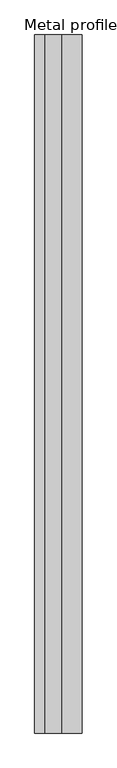
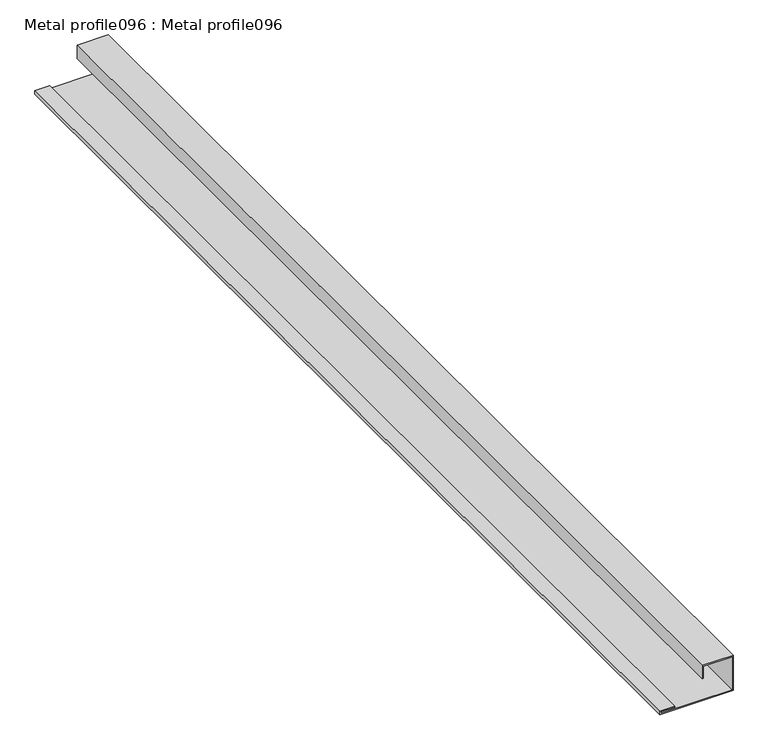
"""IFC4 building model written with IfcOpenShell, lengths in millimetres: proxy geometry, Metal profile096 : Metal profile096."""

import ifcopenshell
import ifcopenshell.guid

model = None  # the IFC model being written
_history = None  # IfcOwnerHistory: only IFC2X3 demands one
_inside = {}  # id of a spatial element -> (the spatial element, [elements in it])
_under = {}  # id of a project, library or spatial element -> (it, [spatial elements below it])
_declared = {}  # id of a project -> (the project, [libraries it declares])
_typed = {}  # id of a type object -> (the type object, [elements of that type])
_made_of = {}  # id of a material, layer set ... -> (it, [elements and type objects made of it])


def new_model(schema):
    """Start an empty IFC model of exactly this schema.

    Asked for "IFC4X3", IfcOpenShell would pick the latest addendum, in which some entities
    have other attributes; the version numbers below select the first issue.
    IFC2X3 requires an IfcOwnerHistory on every rooted entity: one is made here for all.
    """
    global model, _history
    if schema == "IFC4X3":
        model = ifcopenshell.file(schema_version=(4, 3, 0, 0))
    else:
        model = ifcopenshell.file(schema=schema)
    _inside.clear()
    _under.clear()
    _declared.clear()
    _typed.clear()
    _made_of.clear()
    _history = None
    if model.schema == "IFC2X3":
        org = make("IfcOrganization", Name="unknown")
        user = make(
            "IfcPersonAndOrganization",
            ThePerson=make("IfcPerson", FamilyName="unknown"),
            TheOrganization=org,
        )
        app = make(
            "IfcApplication",
            ApplicationDeveloper=org,
            Version="unknown",
            ApplicationFullName="unknown",
            ApplicationIdentifier="unknown",
        )
        _history = make(
            "IfcOwnerHistory",
            OwningUser=user,
            OwningApplication=app,
            ChangeAction="ADDED",
            CreationDate=0,
        )
    return model


def make(cls, **values):
    """One entity of the class cls with the attributes given. An attribute that is None is left unset."""
    return model.create_entity(
        cls, **{name: value for name, value in values.items() if value is not None}
    )


def rooted(cls, **values):
    """An entity with a GlobalId (a new one), such as an element, a storey or a relation."""
    return make(cls, GlobalId=ifcopenshell.guid.new(), OwnerHistory=_history, **values)


def si_unit(unit_type, name, prefix=None):
    """IfcSIUnit, for example si_unit("LENGTHUNIT", "METRE", prefix="MILLI")."""
    return make("IfcSIUnit", UnitType=unit_type, Prefix=prefix, Name=name)


def assignment(units):
    """IfcUnitAssignment: the units of a project."""
    return None if units is None else make("IfcUnitAssignment", Units=units)


def point(xyz):
    """IfcCartesianPoint."""
    return None if xyz is None else make("IfcCartesianPoint", Coordinates=xyz)


def direction(xyz):
    """IfcDirection."""
    return None if xyz is None else make("IfcDirection", DirectionRatios=xyz)


def frame(location, z_axis=None, x_axis=None):
    """IfcAxis2Placement3D, a coordinate frame: its origin and axes. An axis left out is left unset."""
    return make(
        "IfcAxis2Placement3D",
        Location=point(location),
        Axis=direction(z_axis),
        RefDirection=direction(x_axis),
    )


def origin():
    """The frame at (0, 0, 0) with its axes left unset."""
    return frame((0.0, 0.0, 0.0))


def place(relative_to, where):
    """IfcLocalPlacement: puts the frame where relative to a parent placement (None: the world)."""
    return make(
        "IfcLocalPlacement", PlacementRelTo=relative_to, RelativePlacement=where
    )


def context(
    kind, dimensions, precision=None, world=None, true_north=None, identifier=None
):
    """IfcGeometricRepresentationContext, for example the 3D "Model" context."""
    return make(
        "IfcGeometricRepresentationContext",
        ContextIdentifier=identifier,
        ContextType=kind,
        CoordinateSpaceDimension=dimensions,
        Precision=precision,
        WorldCoordinateSystem=world,
        TrueNorth=true_north,
    )


def project(units=None, contexts=None):
    """IfcProject with its units and contexts."""
    return rooted(
        "IfcProject",
        Name="project",
        RepresentationContexts=contexts,
        UnitsInContext=assignment(units),
    )


def spatial(cls, under=None, at=None, **own):
    """A site, building, storey or space (cls), placed at a placement, below another one or the project."""
    s = rooted(cls, ObjectPlacement=at, **own)
    if under is not None:
        _under.setdefault(under.id(), (under, []))[1].append(s)
    return s


def polyline(points):
    """IfcPolyline through the points."""
    return make("IfcPolyline", Points=[point(p) for p in points])


def outline(outer, holes=None, kind="AREA"):
    """IfcArbitraryClosedProfileDef: a profile drawn as a closed curve; with holes, ...WithVoids."""
    if holes is None:
        return make("IfcArbitraryClosedProfileDef", ProfileType=kind, OuterCurve=outer)
    return make(
        "IfcArbitraryProfileDefWithVoids",
        ProfileType=kind,
        OuterCurve=outer,
        InnerCurves=holes,
    )


def extrude(swept, where, along, depth):
    """IfcExtrudedAreaSolid: the profile swept, set in the frame where, extruded along a direction by depth."""
    return make(
        "IfcExtrudedAreaSolid",
        SweptArea=swept,
        Position=where,
        ExtrudedDirection=direction(along),
        Depth=depth,
    )


def shape(context_of_items, identifier, shape_type, items):
    """IfcShapeRepresentation: the items that make up one representation, for example the "Body"."""
    return make(
        "IfcShapeRepresentation",
        ContextOfItems=context_of_items,
        RepresentationIdentifier=identifier,
        RepresentationType=shape_type,
        Items=items,
    )


def source(mapping_origin, context_of_items, identifier, shape_type, items):
    """IfcRepresentationMap: a shape defined once, which mapped items show again and again."""
    return make(
        "IfcRepresentationMap",
        MappingOrigin=mapping_origin,
        MappedRepresentation=shape(context_of_items, identifier, shape_type, items),
    )


def transform(
    local_origin,
    x_axis=None,
    y_axis=None,
    z_axis=None,
    scale=None,
    scale2=None,
    scale3=None,
    uniform=True,
):
    """IfcCartesianTransformationOperator3D, or its non-uniform kind. x_axis, y_axis, z_axis: its Axis1, 2, 3."""
    if uniform:
        return make(
            "IfcCartesianTransformationOperator3D",
            Axis1=direction(x_axis),
            Axis2=direction(y_axis),
            LocalOrigin=point(local_origin),
            Scale=scale,
            Axis3=direction(z_axis),
        )
    return make(
        "IfcCartesianTransformationOperator3DnonUniform",
        Axis1=direction(x_axis),
        Axis2=direction(y_axis),
        LocalOrigin=point(local_origin),
        Scale=scale,
        Axis3=direction(z_axis),
        Scale2=scale2,
        Scale3=scale3,
    )


def mapped(mapping_source, mapping_target):
    """IfcMappedItem: shows the shape of a source again, moved by a transform."""
    return make(
        "IfcMappedItem", MappingSource=mapping_source, MappingTarget=mapping_target
    )


def made_of(thing, what):
    """Note that an element or type object is made of a material, layer set ...; save() writes the relation."""
    if what is not None:
        _made_of.setdefault(what.id(), (what, []))[1].append(thing)
    return thing


def element(
    cls,
    number,
    at=None,
    inside=None,
    cuts=None,
    type_object=None,
    material=None,
    context=None,
    identifier="Body",
    shape_type=None,
    held_by="IfcProductDefinitionShape",
    body=None,
    shapes=None,
    **own,
):
    """One element of the class cls, such as IfcWall. Its Tag is "e" and its number.

    at: its placement. inside: the storey or other place that contains it. cuts: it is an
    opening in that element (IfcRelVoidsElement). A single representation is given by context,
    identifier, shape_type and body (its items); several are given by shapes. held_by: the class
    of the entity that holds the representations. save() writes the other relations.
    """
    e = rooted(cls, Tag="e%d" % number, ObjectPlacement=at, **own)
    if body is not None:
        shapes = [shape(context, identifier, shape_type, body)]
    if shapes is not None:
        e.Representation = make(held_by, Representations=shapes)
    if inside is not None:
        _inside.setdefault(inside.id(), (inside, []))[1].append(e)
    if cuts is not None:
        rooted(
            "IfcRelVoidsElement", RelatingBuildingElement=cuts, RelatedOpeningElement=e
        )
    if type_object is not None:
        _typed.setdefault(type_object.id(), (type_object, []))[1].append(e)
    return made_of(e, material)


def aggregate(whole, parts):
    """IfcRelAggregates: a whole, such as a stair, and the parts it consists of."""
    return rooted("IfcRelAggregates", RelatingObject=whole, RelatedObjects=parts)


def save(model, path):
    """Write the relations noted so far, then the file.

    IfcRelAggregates (storeys below a building ...), IfcRelContainedInSpatialStructure (elements
    in a storey), IfcRelDefinesByType, IfcRelAssociatesMaterial and IfcRelDeclares: one each for
    every whole, place, type object, material and project.
    """
    for whole, parts in _under.values():
        aggregate(whole, parts)
    for where, things in _inside.values():
        rooted(
            "IfcRelContainedInSpatialStructure",
            RelatedElements=things,
            RelatingStructure=where,
        )
    for kind, things in _typed.values():
        rooted("IfcRelDefinesByType", RelatedObjects=things, RelatingType=kind)
    for what, things in _made_of.values():
        rooted("IfcRelAssociatesMaterial", RelatedObjects=things, RelatingMaterial=what)
    for by, libraries in _declared.values():
        rooted("IfcRelDeclares", RelatingContext=by, RelatedDefinitions=libraries)
    model.write(path)


def metal_profile096_metal_profile096_bd596d1d(model_context):
    return source(origin(), model_context, "Body", "SweptSolid", [
        extrude(outline(polyline([(43457.8392595, 17636.3467417), (43459.8392595, 17636.3467417), (43459.8392595, 17608.5835581), (43452.972072, 17608.5835581), (43452.972072, 17744.1826792), (43521.7455095, 17744.1826792), (43521.7455095, 17686.8374644), (43495.6517595, 17686.8374644), (43495.6517595, 17688.8374644), (43519.7455095, 17688.8374644), (43519.7455095, 17742.1826792), (43454.972072, 17742.1826792), (43454.972072, 17610.5835581), (43457.8392595, 17610.5835581), (43457.8392595, 17636.3467417)])), frame((0.0, 7982.1507711, 0.0), z_axis=(0.0, 1.0, 0.0), x_axis=(0.0, 0.0, 1.0)), (0.0, 0.0, 1.0), 2000.0),
    ])


if __name__ == "__main__":
    model = new_model("IFC4")
    model_context = context("Model", 3, world=origin())
    ifc_project = project(units=[si_unit("LENGTHUNIT", "METRE", prefix="MILLI")], contexts=[model_context])
    site = spatial("IfcSite", under=ifc_project)
    building = spatial("IfcBuilding", under=site)
    placement = place(None, origin())
    metal_profile096_metal_profile096_shape = metal_profile096_metal_profile096_bd596d1d(model_context)
    element("IfcBuildingElementProxy", 1, Name="Metal profile096 : Metal profile096", ObjectType="Metal profile096 : Metal profile096", at=placement, inside=building, context=model_context, shape_type="MappedRepresentation", body=[
        mapped(metal_profile096_metal_profile096_shape, transform((0.0, 0.0, 0.0), x_axis=(1.0, 0.0, 0.0), y_axis=(0.0, 1.0, 0.0), z_axis=(0.0, 0.0, 1.0))),
    ])
    save(model, "model.ifc")

# Revit data of these elements
# Type "Metal profile096 : Metal profile096"
#   NameOverride = "Metal profile096"
# Element 1 (IfcBuildingElementProxy, "Metal profile096 : Metal profile096")
#   Materials on its faces: "RECEIVER TRIM 1393"
# Materials
#   "RECEIVER TRIM 1393": class "Unassigned", colour RGB 255 250 0, transparency 0
